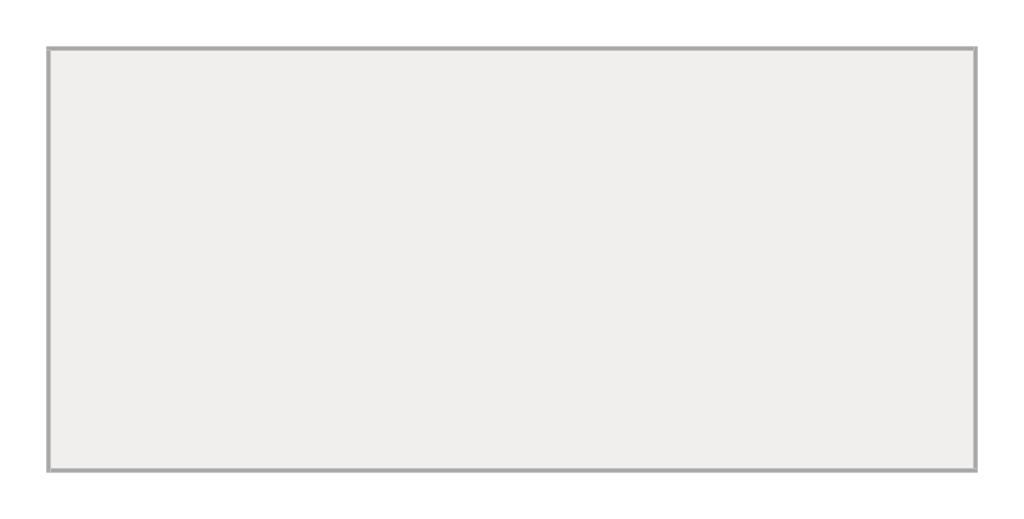
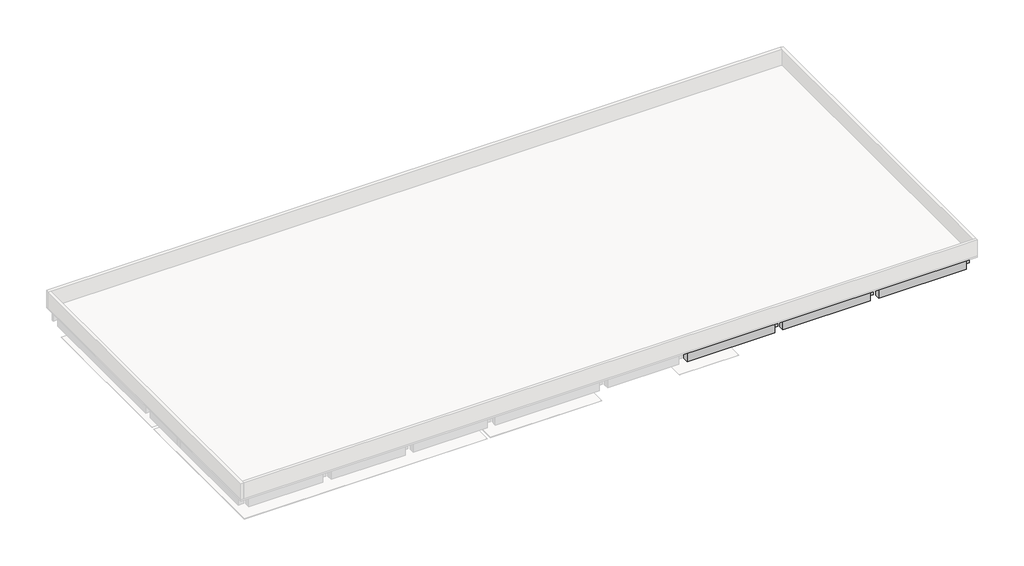
# One storey, part 2 of 2: 34 beams.
"""IFC4 building model written with IfcOpenShell, lengths in millimetres."""

from ifc_helpers import new_model, si_unit, frame, origin, place, context, project, spatial, polyline, outline, extrude, faceted_brep, element, save

model = new_model("IFC4")

# Units and contexts
model_context = context("Model", 3, world=origin())
ifc_project = project(units=[si_unit("LENGTHUNIT", "METRE", prefix="MILLI")], contexts=[model_context])

# Site, building, storey
site = spatial("IfcSite", under=ifc_project)
building = spatial("IfcBuilding", under=site)
storey = spatial("IfcBuildingStorey", under=building, Name="TOC", Elevation=7650.0)

# Beams
placement = place(None, origin())
element("IfcBeam", 1, ObjectType="RC Beam_Rectangular : H_SB_ACB_B400xH900", at=placement, inside=storey, context=model_context, shape_type="Brep", body=[
    faceted_brep([(32124.7, 12116.5208589, 6750.0), (32124.7, 12116.5208589, 7549.0), (31724.7, 12116.5208589, 7549.0), (26324.7, 12116.5208589, 7549.0), (26324.7, 12116.5208589, 6750.0), (31724.7, 12116.5208589, 6750.0), (32124.7, 12516.5208589, 6750.0), (26324.7, 12516.5208589, 6750.0), (31724.7, 12516.5208589, 6750.0), (32124.7, 12516.5208589, 7549.0), (26324.7, 12516.5208589, 7549.0), (31724.7, 12516.5208589, 7549.0)], [[[0, 1, 2, 3, 4, 5]], [[6, 0, 5, 4, 7, 8]], [[9, 6, 8, 7, 10, 11]], [[1, 9, 11, 10, 3, 2]], [[0, 6, 9, 1]], [[4, 3, 10, 7]]]),
])
element("IfcBeam", 2, ObjectType="RC Beam_Rectangular : H_SB_ACB_B400xH900", at=placement, inside=storey, context=model_context, shape_type="Brep", body=[
    faceted_brep([(39124.7, 12116.5208589, 6750.0), (39124.7, 12116.5208589, 7549.0), (38724.7, 12116.5208589, 7549.0), (32124.7, 12116.5208589, 7549.0), (32124.7, 12116.5208589, 6750.0), (38724.7, 12116.5208589, 6750.0), (39124.7, 12516.5208589, 6750.0), (32124.7, 12516.5208589, 6750.0), (38724.7, 12516.5208589, 6750.0), (39124.7, 12516.5208589, 7549.0), (32124.7, 12516.5208589, 7549.0), (38724.7, 12516.5208589, 7549.0)], [[[0, 1, 2, 3, 4, 5]], [[6, 0, 5, 4, 7, 8]], [[9, 6, 8, 7, 10, 11]], [[1, 9, 11, 10, 3, 2]], [[0, 6, 9, 1]], [[4, 3, 10, 7]]]),
])
element("IfcBeam", 3, ObjectType="RC Beam_Rectangular : H_SB_ACB_B400xH900", at=placement, inside=storey, context=model_context, shape_type="Brep", body=[
    faceted_brep([(46124.7, 12116.5208589, 6750.0), (46124.7, 12116.5208589, 7549.0), (45724.7, 12116.5208589, 7549.0), (39124.7, 12116.5208589, 7549.0), (39124.7, 12116.5208589, 6750.0), (45724.7, 12116.5208589, 6750.0), (46124.7, 12516.5208589, 6750.0), (39124.7, 12516.5208589, 6750.0), (45724.7, 12516.5208589, 6750.0), (46124.7, 12516.5208589, 7549.0), (39124.7, 12516.5208589, 7549.0), (45724.7, 12516.5208589, 7549.0)], [[[0, 1, 2, 3, 4, 5]], [[6, 0, 5, 4, 7, 8]], [[9, 6, 8, 7, 10, 11]], [[1, 9, 11, 10, 3, 2]], [[0, 6, 9, 1]], [[4, 3, 10, 7]]]),
])
element("IfcBeam", 4, ObjectType="RC Beam_Rectangular : H_SB_ACB_B400xH900", at=placement, inside=storey, context=model_context, shape_type="Brep", body=[
    faceted_brep([(53124.7, 12116.5208589, 6750.0), (53124.7, 12116.5208589, 7549.0), (52724.7, 12116.5208589, 7549.0), (46124.7, 12116.5208589, 7549.0), (46124.7, 12116.5208589, 6750.0), (52724.7, 12116.5208589, 6750.0), (53124.7, 12516.5208589, 6750.0), (46124.7, 12516.5208589, 6750.0), (52724.7, 12516.5208589, 6750.0), (53124.7, 12516.5208589, 7549.0), (46124.7, 12516.5208589, 7549.0), (52724.7, 12516.5208589, 7549.0)], [[[0, 1, 2, 3, 4, 5]], [[6, 0, 5, 4, 7, 8]], [[9, 6, 8, 7, 10, 11]], [[1, 9, 11, 10, 3, 2]], [[0, 6, 9, 1]], [[4, 3, 10, 7]]]),
])
element("IfcBeam", 5, ObjectType="RC Beam_Rectangular : H_SB_ACB_B400xH900", at=placement, inside=storey, context=model_context, shape_type="SweptSolid", body=[
    extrude(outline(polyline([(7500.0, 224.7), (6750.0, 224.7), (6750.0, 5624.7), (7500.0, 5624.7), (7500.0, 5724.7), (7549.0, 5724.7), (7549.0, 124.7), (7500.0, 124.7), (7500.0, 224.7)])), frame((0.0, 23816.5208589, 0.0), z_axis=(0.0, 1.0, 0.0), x_axis=(0.0, 0.0, 1.0)), (0.0, 0.0, 1.0), 400.0),
])
element("IfcBeam", 6, ObjectType="RC Beam_Rectangular : H_SB_ACB_B400xH900", at=placement, inside=storey, context=model_context, shape_type="SweptSolid", body=[
    extrude(outline(polyline([(7500.0, 6224.7), (6750.0, 6224.7), (6750.0, 11624.7), (7500.0, 11624.7), (7500.0, 11724.7), (7549.0, 11724.7), (7549.0, 6124.7), (7500.0, 6124.7), (7500.0, 6224.7)])), frame((0.0, 23816.5208589, 0.0), z_axis=(0.0, 1.0, 0.0), x_axis=(0.0, 0.0, 1.0)), (0.0, 0.0, 1.0), 400.0),
])
element("IfcBeam", 7, ObjectType="RC Beam_Rectangular : H_SB_ACB_B400xH900", at=placement, inside=storey, context=model_context, shape_type="SweptSolid", body=[
    extrude(outline(polyline([(7500.0, 12224.7), (6750.0, 12224.7), (6750.0, 17624.7), (7500.0, 17624.7), (7500.0, 17724.7), (7549.0, 17724.7), (7549.0, 12124.7), (7500.0, 12124.7), (7500.0, 12224.7)])), frame((0.0, 23816.5208589, 0.0), z_axis=(0.0, 1.0, 0.0), x_axis=(0.0, 0.0, 1.0)), (0.0, 0.0, 1.0), 400.0),
])
element("IfcBeam", 8, ObjectType="RC Beam_Rectangular : H_SB_ACB_B400xH900", at=placement, inside=storey, context=model_context, shape_type="SweptSolid", body=[
    extrude(outline(polyline([(7500.0, 18224.7), (6750.0, 18224.7), (6750.0, 25824.7), (7500.0, 25824.7), (7500.0, 25924.7), (7549.0, 25924.7), (7549.0, 18124.7), (7500.0, 18124.7), (7500.0, 18224.7)])), frame((0.0, 23816.5208589, 0.0), z_axis=(0.0, 1.0, 0.0), x_axis=(0.0, 0.0, 1.0)), (0.0, 0.0, 1.0), 400.0),
])
element("IfcBeam", 9, ObjectType="RC Beam_Rectangular : H_SB_ACB_B400xH900", at=placement, inside=storey, context=model_context, shape_type="SweptSolid", body=[
    extrude(outline(polyline([(7500.0, 26424.7), (6750.0, 26424.7), (6750.0, 31624.7), (7500.0, 31624.7), (7500.0, 31724.7), (7549.0, 31724.7), (7549.0, 26324.7), (7500.0, 26324.7), (7500.0, 26424.7)])), frame((0.0, 23816.5208589, 0.0), z_axis=(0.0, 1.0, 0.0), x_axis=(0.0, 0.0, 1.0)), (0.0, 0.0, 1.0), 400.0),
])
element("IfcBeam", 10, ObjectType="RC Beam_Rectangular : H_SB_ACB_B400xH900", at=placement, inside=storey, context=model_context, shape_type="SweptSolid", body=[
    extrude(outline(polyline([(7500.0, 32224.7), (6750.0, 32224.7), (6750.0, 38624.7), (7500.0, 38624.7), (7500.0, 38724.7), (7549.0, 38724.7), (7549.0, 32124.7), (7500.0, 32124.7), (7500.0, 32224.7)])), frame((0.0, 23816.5208589, 0.0), z_axis=(0.0, 1.0, 0.0), x_axis=(0.0, 0.0, 1.0)), (0.0, 0.0, 1.0), 400.0),
])
element("IfcBeam", 11, ObjectType="RC Beam_Rectangular : H_SB_ACB_B400xH900", at=placement, inside=storey, context=model_context, shape_type="SweptSolid", body=[
    extrude(outline(polyline([(7500.0, 39224.7), (6750.0, 39224.7), (6750.0, 45624.7), (7500.0, 45624.7), (7500.0, 45724.7), (7549.0, 45724.7), (7549.0, 39124.7), (7500.0, 39124.7), (7500.0, 39224.7)])), frame((0.0, 23816.5208589, 0.0), z_axis=(0.0, 1.0, 0.0), x_axis=(0.0, 0.0, 1.0)), (0.0, 0.0, 1.0), 400.0),
])
element("IfcBeam", 12, ObjectType="RC Beam_Rectangular : H_SB_ACB_B400xH900", at=placement, inside=storey, context=model_context, shape_type="SweptSolid", body=[
    extrude(outline(polyline([(7500.0, 46224.7), (6750.0, 46224.7), (6750.0, 52624.7), (7500.0, 52624.7), (7500.0, 52724.7), (7549.0, 52724.7), (7549.0, 46124.7), (7500.0, 46124.7), (7500.0, 46224.7)])), frame((0.0, 23816.5208589, 0.0), z_axis=(0.0, 1.0, 0.0), x_axis=(0.0, 0.0, 1.0)), (0.0, 0.0, 1.0), 400.0),
])
element("IfcBeam", 13, ObjectType="RC Beam_Rectangular : H_SB_ACB_B400xH900", at=placement, inside=storey, context=model_context, shape_type="Brep", body=[
    faceted_brep([(26424.7, 8216.5208589, 7500.0), (26424.7, 8216.5208589, 6750.0), (31624.7, 8216.5208589, 6750.0), (31624.7, 8216.5208589, 7500.0), (31724.7, 8216.5208589, 7500.0), (32124.7, 8216.5208589, 7500.0), (32124.7, 8216.5208589, 7549.0), (31724.7, 8216.5208589, 7549.0), (26324.7, 8216.5208589, 7549.0), (26324.7, 8216.5208589, 7500.0), (26424.7, 8616.5208589, 6750.0), (31624.7, 8616.5208589, 6750.0), (26424.7, 8616.5208589, 7500.0), (26324.7, 8616.5208589, 7500.0), (26324.7, 8616.5208589, 7549.0), (31724.7, 8616.5208589, 7549.0), (32124.7, 8616.5208589, 7549.0), (32124.7, 8616.5208589, 7500.0), (31724.7, 8616.5208589, 7500.0), (31624.7, 8616.5208589, 7500.0)], [[[0, 1, 2, 3, 4, 5, 6, 7, 8, 9]], [[1, 10, 11, 2]], [[10, 12, 13, 14, 15, 16, 17, 18, 19, 11]], [[1, 0, 12, 10]], [[0, 9, 13, 12]], [[19, 3, 2, 11]], [[3, 19, 18, 17, 5, 4]], [[8, 7, 6, 16, 15, 14]], [[16, 6, 5, 17]], [[8, 14, 13, 9]]]),
])
element("IfcBeam", 14, ObjectType="RC Beam_Rectangular : H_SB_ACB_B400xH900", at=placement, inside=storey, context=model_context, shape_type="Brep", body=[
    faceted_brep([(32224.7, 8216.5208589, 7500.0), (32224.7, 8216.5208589, 6750.0), (38624.7, 8216.5208589, 6750.0), (38624.7, 8216.5208589, 7500.0), (38724.7, 8216.5208589, 7500.0), (39124.7, 8216.5208589, 7500.0), (39124.7, 8216.5208589, 7549.0), (38724.7, 8216.5208589, 7549.0), (32124.7, 8216.5208589, 7549.0), (32124.7, 8216.5208589, 7500.0), (32224.7, 8616.5208589, 6750.0), (38624.7, 8616.5208589, 6750.0), (32224.7, 8616.5208589, 7500.0), (32124.7, 8616.5208589, 7500.0), (32124.7, 8616.5208589, 7549.0), (38724.7, 8616.5208589, 7549.0), (39124.7, 8616.5208589, 7549.0), (39124.7, 8616.5208589, 7500.0), (38724.7, 8616.5208589, 7500.0), (38624.7, 8616.5208589, 7500.0)], [[[0, 1, 2, 3, 4, 5, 6, 7, 8, 9]], [[1, 10, 11, 2]], [[10, 12, 13, 14, 15, 16, 17, 18, 19, 11]], [[1, 0, 12, 10]], [[0, 9, 13, 12]], [[19, 3, 2, 11]], [[3, 19, 18, 17, 5, 4]], [[8, 7, 6, 16, 15, 14]], [[16, 6, 5, 17]], [[8, 14, 13, 9]]]),
])
element("IfcBeam", 15, ObjectType="RC Beam_Rectangular : H_SB_ACB_B400xH900", at=placement, inside=storey, context=model_context, shape_type="Brep", body=[
    faceted_brep([(39224.7, 8216.5208589, 7500.0), (39224.7, 8216.5208589, 6750.0), (45624.7, 8216.5208589, 6750.0), (45624.7, 8216.5208589, 7500.0), (45724.7, 8216.5208589, 7500.0), (46124.7, 8216.5208589, 7500.0), (46124.7, 8216.5208589, 7549.0), (45724.7, 8216.5208589, 7549.0), (39124.7, 8216.5208589, 7549.0), (39124.7, 8216.5208589, 7500.0), (39224.7, 8616.5208589, 6750.0), (45624.7, 8616.5208589, 6750.0), (39224.7, 8616.5208589, 7500.0), (39124.7, 8616.5208589, 7500.0), (39124.7, 8616.5208589, 7549.0), (45724.7, 8616.5208589, 7549.0), (46124.7, 8616.5208589, 7549.0), (46124.7, 8616.5208589, 7500.0), (45724.7, 8616.5208589, 7500.0), (45624.7, 8616.5208589, 7500.0)], [[[0, 1, 2, 3, 4, 5, 6, 7, 8, 9]], [[1, 10, 11, 2]], [[10, 12, 13, 14, 15, 16, 17, 18, 19, 11]], [[1, 0, 12, 10]], [[0, 9, 13, 12]], [[19, 3, 2, 11]], [[3, 19, 18, 17, 5, 4]], [[8, 7, 6, 16, 15, 14]], [[16, 6, 5, 17]], [[8, 14, 13, 9]]]),
])
element("IfcBeam", 16, ObjectType="RC Beam_Rectangular : H_SB_ACB_B400xH900", at=placement, inside=storey, context=model_context, shape_type="Brep", body=[
    faceted_brep([(46224.7, 8216.5208589, 7500.0), (46224.7, 8216.5208589, 6750.0), (52624.7, 8216.5208589, 6750.0), (52624.7, 8216.5208589, 7500.0), (52724.7, 8216.5208589, 7500.0), (53124.7, 8216.5208589, 7500.0), (53124.7, 8216.5208589, 7549.0), (52724.7, 8216.5208589, 7549.0), (46124.7, 8216.5208589, 7549.0), (46124.7, 8216.5208589, 7500.0), (46224.7, 8616.5208589, 6750.0), (52624.7, 8616.5208589, 6750.0), (46224.7, 8616.5208589, 7500.0), (46124.7, 8616.5208589, 7500.0), (46124.7, 8616.5208589, 7549.0), (52724.7, 8616.5208589, 7549.0), (53124.7, 8616.5208589, 7549.0), (53124.7, 8616.5208589, 7500.0), (52724.7, 8616.5208589, 7500.0), (52624.7, 8616.5208589, 7500.0)], [[[0, 1, 2, 3, 4, 5, 6, 7, 8, 9]], [[1, 10, 11, 2]], [[10, 12, 13, 14, 15, 16, 17, 18, 19, 11]], [[1, 0, 12, 10]], [[0, 9, 13, 12]], [[19, 3, 2, 11]], [[3, 19, 18, 17, 5, 4]], [[8, 7, 6, 16, 15, 14]], [[16, 6, 5, 17]], [[8, 14, 13, 9]]]),
])
element("IfcBeam", 17, ObjectType="RC Beam_Rectangular : H_SB_ACB_B400xH900", at=placement, inside=storey, context=model_context, shape_type="Brep", body=[
    faceted_brep([(32224.7, 416.5208589, 7500.0), (32224.7, 416.5208589, 6750.0), (38624.7, 416.5208589, 6750.0), (38624.7, 416.5208589, 7500.0), (39124.7, 416.5208589, 7500.0), (39124.7, 416.5208589, 7549.0), (32124.7, 416.5208589, 7549.0), (32124.7, 416.5208589, 7500.0), (32224.7, 816.5208589, 6750.0), (38624.7, 816.5208589, 6750.0), (32224.7, 816.5208589, 7500.0), (32124.7, 816.5208589, 7500.0), (32124.7, 816.5208589, 7549.0), (38724.7, 816.5208589, 7549.0), (39124.7, 816.5208589, 7549.0), (39124.7, 816.5208589, 7500.0), (38724.7, 816.5208589, 7500.0), (38624.7, 816.5208589, 7500.0)], [[[0, 1, 2, 3, 4, 5, 6, 7]], [[1, 8, 9, 2]], [[8, 10, 11, 12, 13, 14, 15, 16, 17, 9]], [[8, 1, 0, 10]], [[11, 10, 0, 7]], [[17, 3, 2, 9]], [[3, 17, 16, 15, 4]], [[6, 5, 14, 13, 12]], [[14, 5, 4, 15]], [[6, 12, 11, 7]]]),
])
element("IfcBeam", 18, ObjectType="RC Beam_Rectangular : H_SB_ACB_B400xH900", at=placement, inside=storey, context=model_context, shape_type="Brep", body=[
    faceted_brep([(39224.7, 416.5208589, 7500.0), (39224.7, 416.5208589, 6750.0), (45624.7, 416.5208589, 6750.0), (45624.7, 416.5208589, 7500.0), (46124.7, 416.5208589, 7500.0), (46124.7, 416.5208589, 7549.0), (39124.7, 416.5208589, 7549.0), (39124.7, 416.5208589, 7500.0), (39224.7, 816.5208589, 6750.0), (45624.7, 816.5208589, 6750.0), (39224.7, 816.5208589, 7500.0), (39124.7, 816.5208589, 7500.0), (39124.7, 816.5208589, 7549.0), (45724.7, 816.5208589, 7549.0), (46124.7, 816.5208589, 7549.0), (46124.7, 816.5208589, 7500.0), (45724.7, 816.5208589, 7500.0), (45624.7, 816.5208589, 7500.0)], [[[0, 1, 2, 3, 4, 5, 6, 7]], [[1, 8, 9, 2]], [[8, 10, 11, 12, 13, 14, 15, 16, 17, 9]], [[8, 1, 0, 10]], [[11, 10, 0, 7]], [[17, 3, 2, 9]], [[3, 17, 16, 15, 4]], [[6, 5, 14, 13, 12]], [[14, 5, 4, 15]], [[6, 12, 11, 7]]]),
])
element("IfcBeam", 19, ObjectType="RC Beam_Rectangular : H_SB_ACB_B400xH900", at=placement, inside=storey, context=model_context, shape_type="Brep", body=[
    faceted_brep([(46224.7, 416.5208589, 7500.0), (46224.7, 416.5208589, 6750.0), (52624.7, 416.5208589, 6750.0), (52624.7, 416.5208589, 7500.0), (53124.7, 416.5208589, 7500.0), (53124.7, 416.5208589, 7549.0), (46124.7, 416.5208589, 7549.0), (46124.7, 416.5208589, 7500.0), (46224.7, 816.5208589, 6750.0), (52624.7, 816.5208589, 6750.0), (46224.7, 816.5208589, 7500.0), (46124.7, 816.5208589, 7500.0), (46124.7, 816.5208589, 7549.0), (52724.7, 816.5208589, 7549.0), (53124.7, 816.5208589, 7549.0), (53124.7, 816.5208589, 7500.0), (52724.7, 816.5208589, 7500.0), (52624.7, 816.5208589, 7500.0)], [[[0, 1, 2, 3, 4, 5, 6, 7]], [[1, 8, 9, 2]], [[8, 10, 11, 12, 13, 14, 15, 16, 17, 9]], [[8, 1, 0, 10]], [[11, 10, 0, 7]], [[17, 3, 2, 9]], [[3, 17, 16, 15, 4]], [[6, 5, 14, 13, 12]], [[14, 5, 4, 15]], [[6, 12, 11, 7]]]),
])
element("IfcBeam", 20, ObjectType="RC Beam_Rectangular : H_SB_ACB_B400xH900", at=placement, inside=storey, context=model_context, shape_type="Brep", body=[
    faceted_brep([(6124.7, 24429.2208589, 6750.0), (5724.7, 24429.2208589, 6750.0), (5724.7, 24429.2208589, 7549.0), (6124.7, 24429.2208589, 7549.0), (6124.7, 12616.5208589, 7500.0), (6124.7, 12616.5208589, 6750.0), (6124.7, 23716.5208589, 6750.0), (6124.7, 23716.5208589, 7500.0), (6124.7, 23816.5208589, 7500.0), (6124.7, 24216.5208589, 7500.0), (6124.7, 24316.5208589, 7500.0), (6124.7, 24316.5208589, 6750.0), (6124.7, 24216.5208589, 7549.0), (6124.7, 23816.5208589, 7549.0), (6124.7, 12516.5208589, 7549.0), (6124.7, 12516.5208589, 7500.0), (5724.7, 24316.5208589, 6750.0), (5724.7, 24316.5208589, 7500.0), (5724.7, 24216.5208589, 7500.0), (5724.7, 23816.5208589, 7500.0), (5724.7, 23716.5208589, 7500.0), (5724.7, 23716.5208589, 6750.0), (5724.7, 12616.5208589, 6750.0), (5724.7, 12616.5208589, 7500.0), (5724.7, 12516.5208589, 7500.0), (5724.7, 12516.5208589, 7549.0), (5724.7, 23816.5208589, 7549.0), (5724.7, 24216.5208589, 7549.0)], [[[0, 1, 2, 3]], [[4, 5, 6, 7, 8, 9, 10, 11, 0, 3, 12, 13, 14, 15]], [[1, 0, 11, 16]], [[2, 1, 16, 17, 18, 19, 20, 21, 22, 23, 24, 25, 26, 27]], [[24, 15, 14, 25]], [[5, 4, 23, 22]], [[4, 15, 24, 23]], [[20, 7, 6, 21]], [[7, 20, 19, 18, 17, 10, 9, 8]], [[3, 2, 27, 26, 25, 14, 13, 12]], [[10, 17, 16, 11]], [[5, 22, 21, 6]]]),
])
element("IfcBeam", 21, ObjectType="RC Beam_Rectangular : H_SB_ACB_B400xH900", at=placement, inside=storey, context=model_context, shape_type="Brep", body=[
    faceted_brep([(12124.7, 24429.2208589, 6750.0), (11724.7, 24429.2208589, 6750.0), (11724.7, 24429.2208589, 7549.0), (12124.7, 24429.2208589, 7549.0), (12124.7, 12616.5208589, 7500.0), (12124.7, 12616.5208589, 6750.0), (12124.7, 23716.5208589, 6750.0), (12124.7, 23716.5208589, 7500.0), (12124.7, 23816.5208589, 7500.0), (12124.7, 24216.5208589, 7500.0), (12124.7, 24316.5208589, 7500.0), (12124.7, 24316.5208589, 6750.0), (12124.7, 24216.5208589, 7549.0), (12124.7, 23816.5208589, 7549.0), (12124.7, 12516.5208589, 7549.0), (12124.7, 12516.5208589, 7500.0), (11724.7, 24316.5208589, 6750.0), (11724.7, 24316.5208589, 7500.0), (11724.7, 24216.5208589, 7500.0), (11724.7, 23816.5208589, 7500.0), (11724.7, 23716.5208589, 7500.0), (11724.7, 23716.5208589, 6750.0), (11724.7, 12616.5208589, 6750.0), (11724.7, 12616.5208589, 7500.0), (11724.7, 12516.5208589, 7500.0), (11724.7, 12516.5208589, 7549.0), (11724.7, 23816.5208589, 7549.0), (11724.7, 24216.5208589, 7549.0)], [[[0, 1, 2, 3]], [[4, 5, 6, 7, 8, 9, 10, 11, 0, 3, 12, 13, 14, 15]], [[1, 0, 11, 16]], [[2, 1, 16, 17, 18, 19, 20, 21, 22, 23, 24, 25, 26, 27]], [[24, 15, 14, 25]], [[5, 4, 23, 22]], [[4, 15, 24, 23]], [[20, 7, 6, 21]], [[7, 20, 19, 18, 17, 10, 9, 8]], [[3, 2, 27, 26, 25, 14, 13, 12]], [[10, 17, 16, 11]], [[5, 22, 21, 6]]]),
])
element("IfcBeam", 22, ObjectType="RC Beam_Rectangular : H_SB_ACB_B400xH900", at=placement, inside=storey, context=model_context, shape_type="Brep", body=[
    faceted_brep([(18124.7, 24429.2208589, 6750.0), (17724.7, 24429.2208589, 6750.0), (17724.7, 24429.2208589, 7549.0), (18124.7, 24429.2208589, 7549.0), (18124.7, 12616.5208589, 7500.0), (18124.7, 12616.5208589, 6750.0), (18124.7, 23716.5208589, 6750.0), (18124.7, 23716.5208589, 7500.0), (18124.7, 23816.5208589, 7500.0), (18124.7, 24216.5208589, 7500.0), (18124.7, 24316.5208589, 7500.0), (18124.7, 24316.5208589, 6750.0), (18124.7, 24216.5208589, 7549.0), (18124.7, 23816.5208589, 7549.0), (18124.7, 12516.5208589, 7549.0), (18124.7, 12516.5208589, 7500.0), (17724.7, 24316.5208589, 6750.0), (17724.7, 24316.5208589, 7500.0), (17724.7, 24216.5208589, 7500.0), (17724.7, 23816.5208589, 7500.0), (17724.7, 23716.5208589, 7500.0), (17724.7, 23716.5208589, 6750.0), (17724.7, 12616.5208589, 6750.0), (17724.7, 12616.5208589, 7500.0), (17724.7, 12516.5208589, 7500.0), (17724.7, 12516.5208589, 7549.0), (17724.7, 23816.5208589, 7549.0), (17724.7, 24216.5208589, 7549.0)], [[[0, 1, 2, 3]], [[4, 5, 6, 7, 8, 9, 10, 11, 0, 3, 12, 13, 14, 15]], [[1, 0, 11, 16]], [[2, 1, 16, 17, 18, 19, 20, 21, 22, 23, 24, 25, 26, 27]], [[24, 15, 14, 25]], [[5, 4, 23, 22]], [[4, 15, 24, 23]], [[20, 7, 6, 21]], [[7, 20, 19, 18, 17, 10, 9, 8]], [[3, 2, 27, 26, 25, 14, 13, 12]], [[10, 17, 16, 11]], [[5, 22, 21, 6]]]),
])
element("IfcBeam", 23, ObjectType="RC Beam_Rectangular : H_SB_ACB_B400xH900", at=placement, inside=storey, context=model_context, shape_type="Brep", body=[
    faceted_brep([(26324.7, 24429.2208589, 6750.0), (25924.7, 24429.2208589, 6750.0), (25924.7, 24429.2208589, 7549.0), (26324.7, 24429.2208589, 7549.0), (26324.7, 24216.5208589, 7549.0), (26324.7, 23816.5208589, 7549.0), (26324.7, 12516.5208589, 7549.0), (26324.7, 12516.5208589, 6750.0), (26324.7, 23716.5208589, 6750.0), (26324.7, 23716.5208589, 7500.0), (26324.7, 23816.5208589, 7500.0), (26324.7, 24216.5208589, 7500.0), (26324.7, 24316.5208589, 7500.0), (26324.7, 24316.5208589, 6750.0), (25924.7, 24316.5208589, 6750.0), (25924.7, 12516.5208589, 6750.0), (25924.7, 12516.5208589, 7549.0), (25924.7, 23816.5208589, 7549.0), (25924.7, 24216.5208589, 7549.0), (25924.7, 24316.5208589, 7500.0), (25924.7, 24216.5208589, 7500.0), (25924.7, 23816.5208589, 7500.0), (25924.7, 23716.5208589, 7500.0), (25924.7, 23716.5208589, 6750.0)], [[[0, 1, 2, 3]], [[0, 3, 4, 5, 6, 7, 8, 9, 10, 11, 12, 13]], [[1, 0, 13, 14]], [[15, 16, 17, 18, 2, 1, 14, 19, 20, 21, 22, 23]], [[15, 7, 6, 16]], [[22, 9, 8, 23]], [[9, 22, 21, 20, 19, 12, 11, 10]], [[3, 2, 18, 17, 16, 6, 5, 4]], [[12, 19, 14, 13]], [[7, 15, 23, 8]]]),
])
element("IfcBeam", 24, ObjectType="RC Beam_Rectangular : H_SB_ACB_B400xH900", at=placement, inside=storey, context=model_context, shape_type="SweptSolid", body=[
    extrude(outline(polyline([(12116.5208589, 7549.0), (12116.5208589, 6750.0), (8716.5208589, 6750.0), (8716.5208589, 7500.0), (8616.5208589, 7500.0), (8616.5208589, 7549.0), (12116.5208589, 7549.0)])), frame((31724.7, 0.0, 0.0), z_axis=(1.0, 0.0, 0.0), x_axis=(0.0, 1.0, 0.0)), (0.0, 0.0, 1.0), 400.0),
])
element("IfcBeam", 25, ObjectType="RC Beam_Rectangular : H_SB_ACB_B400xH900", at=placement, inside=storey, context=model_context, shape_type="Brep", body=[
    faceted_brep([(32124.7, 24429.2208589, 6750.0), (31724.7, 24429.2208589, 6750.0), (31724.7, 24429.2208589, 7549.0), (32124.7, 24429.2208589, 7549.0), (32124.7, 24216.5208589, 7549.0), (32124.7, 23816.5208589, 7549.0), (32124.7, 12516.5208589, 7549.0), (32124.7, 12516.5208589, 6750.0), (32124.7, 23716.5208589, 6750.0), (32124.7, 23716.5208589, 7500.0), (32124.7, 23816.5208589, 7500.0), (32124.7, 24216.5208589, 7500.0), (32124.7, 24316.5208589, 7500.0), (32124.7, 24316.5208589, 6750.0), (31724.7, 24316.5208589, 6750.0), (31724.7, 12516.5208589, 6750.0), (31724.7, 12516.5208589, 7549.0), (31724.7, 23816.5208589, 7549.0), (31724.7, 24216.5208589, 7549.0), (31724.7, 24316.5208589, 7500.0), (31724.7, 24216.5208589, 7500.0), (31724.7, 23816.5208589, 7500.0), (31724.7, 23716.5208589, 7500.0), (31724.7, 23716.5208589, 6750.0)], [[[0, 1, 2, 3]], [[0, 3, 4, 5, 6, 7, 8, 9, 10, 11, 12, 13]], [[1, 0, 13, 14]], [[15, 16, 17, 18, 2, 1, 14, 19, 20, 21, 22, 23]], [[15, 7, 6, 16]], [[22, 9, 8, 23]], [[9, 22, 21, 20, 19, 12, 11, 10]], [[3, 2, 18, 17, 16, 6, 5, 4]], [[12, 19, 14, 13]], [[7, 15, 23, 8]]]),
])
element("IfcBeam", 26, ObjectType="RC Beam_Rectangular : H_SB_ACB_B400xH900", at=placement, inside=storey, context=model_context, shape_type="SweptSolid", body=[
    extrude(outline(polyline([(8116.5208589, 7500.0), (8116.5208589, 6750.0), (916.5208589, 6750.0), (916.5208589, 7500.0), (816.5208589, 7500.0), (816.5208589, 7549.0), (8216.5208589, 7549.0), (8216.5208589, 7500.0), (8116.5208589, 7500.0)])), frame((38724.7, 0.0, 0.0), z_axis=(1.0, 0.0, 0.0), x_axis=(0.0, 1.0, 0.0)), (0.0, 0.0, 1.0), 400.0),
])
element("IfcBeam", 27, ObjectType="RC Beam_Rectangular : H_SB_ACB_B400xH900", at=placement, inside=storey, context=model_context, shape_type="SweptSolid", body=[
    extrude(outline(polyline([(12116.5208589, 7549.0), (12116.5208589, 6750.0), (8716.5208589, 6750.0), (8716.5208589, 7500.0), (8616.5208589, 7500.0), (8616.5208589, 7549.0), (12116.5208589, 7549.0)])), frame((38724.7, 0.0, 0.0), z_axis=(1.0, 0.0, 0.0), x_axis=(0.0, 1.0, 0.0)), (0.0, 0.0, 1.0), 400.0),
])
element("IfcBeam", 28, ObjectType="RC Beam_Rectangular : H_SB_ACB_B400xH900", at=placement, inside=storey, context=model_context, shape_type="Brep", body=[
    faceted_brep([(39124.7, 24429.2208589, 6750.0), (38724.7, 24429.2208589, 6750.0), (38724.7, 24429.2208589, 7549.0), (39124.7, 24429.2208589, 7549.0), (39124.7, 24216.5208589, 7549.0), (39124.7, 23816.5208589, 7549.0), (39124.7, 12516.5208589, 7549.0), (39124.7, 12516.5208589, 6750.0), (39124.7, 23716.5208589, 6750.0), (39124.7, 23716.5208589, 7500.0), (39124.7, 23816.5208589, 7500.0), (39124.7, 24216.5208589, 7500.0), (39124.7, 24316.5208589, 7500.0), (39124.7, 24316.5208589, 6750.0), (38724.7, 24316.5208589, 6750.0), (38724.7, 12516.5208589, 6750.0), (38724.7, 12516.5208589, 7549.0), (38724.7, 23816.5208589, 7549.0), (38724.7, 24216.5208589, 7549.0), (38724.7, 24316.5208589, 7500.0), (38724.7, 24216.5208589, 7500.0), (38724.7, 23816.5208589, 7500.0), (38724.7, 23716.5208589, 7500.0), (38724.7, 23716.5208589, 6750.0)], [[[0, 1, 2, 3]], [[0, 3, 4, 5, 6, 7, 8, 9, 10, 11, 12, 13]], [[1, 0, 13, 14]], [[15, 16, 17, 18, 2, 1, 14, 19, 20, 21, 22, 23]], [[15, 7, 6, 16]], [[22, 9, 8, 23]], [[9, 22, 21, 20, 19, 12, 11, 10]], [[3, 2, 18, 17, 16, 6, 5, 4]], [[12, 19, 14, 13]], [[7, 15, 23, 8]]]),
])
element("IfcBeam", 29, ObjectType="RC Beam_Rectangular : H_SB_ACB_B400xH900", at=placement, inside=storey, context=model_context, shape_type="SweptSolid", body=[
    extrude(outline(polyline([(8116.5208589, 7500.0), (8116.5208589, 6750.0), (916.5208589, 6750.0), (916.5208589, 7500.0), (816.5208589, 7500.0), (816.5208589, 7549.0), (8216.5208589, 7549.0), (8216.5208589, 7500.0), (8116.5208589, 7500.0)])), frame((45724.7, 0.0, 0.0), z_axis=(1.0, 0.0, 0.0), x_axis=(0.0, 1.0, 0.0)), (0.0, 0.0, 1.0), 400.0),
])
element("IfcBeam", 30, ObjectType="RC Beam_Rectangular : H_SB_ACB_B400xH900", at=placement, inside=storey, context=model_context, shape_type="SweptSolid", body=[
    extrude(outline(polyline([(12116.5208589, 7549.0), (12116.5208589, 6750.0), (8716.5208589, 6750.0), (8716.5208589, 7500.0), (8616.5208589, 7500.0), (8616.5208589, 7549.0), (12116.5208589, 7549.0)])), frame((45724.7, 0.0, 0.0), z_axis=(1.0, 0.0, 0.0), x_axis=(0.0, 1.0, 0.0)), (0.0, 0.0, 1.0), 400.0),
])
element("IfcBeam", 31, ObjectType="RC Beam_Rectangular : H_SB_ACB_B400xH900", at=placement, inside=storey, context=model_context, shape_type="Brep", body=[
    faceted_brep([(46124.7, 24429.2208589, 6750.0), (45724.7, 24429.2208589, 6750.0), (45724.7, 24429.2208589, 7549.0), (46124.7, 24429.2208589, 7549.0), (46124.7, 24216.5208589, 7549.0), (46124.7, 23816.5208589, 7549.0), (46124.7, 12516.5208589, 7549.0), (46124.7, 12516.5208589, 6750.0), (46124.7, 23716.5208589, 6750.0), (46124.7, 23716.5208589, 7500.0), (46124.7, 23816.5208589, 7500.0), (46124.7, 24216.5208589, 7500.0), (46124.7, 24316.5208589, 7500.0), (46124.7, 24316.5208589, 6750.0), (45724.7, 24316.5208589, 6750.0), (45724.7, 12516.5208589, 6750.0), (45724.7, 12516.5208589, 7549.0), (45724.7, 23816.5208589, 7549.0), (45724.7, 24216.5208589, 7549.0), (45724.7, 24316.5208589, 7500.0), (45724.7, 24216.5208589, 7500.0), (45724.7, 23816.5208589, 7500.0), (45724.7, 23716.5208589, 7500.0), (45724.7, 23716.5208589, 6750.0)], [[[0, 1, 2, 3]], [[0, 3, 4, 5, 6, 7, 8, 9, 10, 11, 12, 13]], [[1, 0, 13, 14]], [[15, 16, 17, 18, 2, 1, 14, 19, 20, 21, 22, 23]], [[15, 7, 6, 16]], [[22, 9, 8, 23]], [[9, 22, 21, 20, 19, 12, 11, 10]], [[3, 2, 18, 17, 16, 6, 5, 4]], [[12, 19, 14, 13]], [[7, 15, 23, 8]]]),
])
element("IfcBeam", 32, ObjectType="RC Beam_Rectangular : H_SB_ACB_B400xH900", at=placement, inside=storey, context=model_context, shape_type="SweptSolid", body=[
    extrude(outline(polyline([(8116.5208589, 7500.0), (8116.5208589, 6750.0), (916.5208589, 6750.0), (916.5208589, 7500.0), (816.5208589, 7500.0), (816.5208589, 7549.0), (8216.5208589, 7549.0), (8216.5208589, 7500.0), (8116.5208589, 7500.0)])), frame((52724.7, 0.0, 0.0), z_axis=(1.0, 0.0, 0.0), x_axis=(0.0, 1.0, 0.0)), (0.0, 0.0, 1.0), 400.0),
])
element("IfcBeam", 33, ObjectType="RC Beam_Rectangular : H_SB_ACB_B400xH900", at=placement, inside=storey, context=model_context, shape_type="SweptSolid", body=[
    extrude(outline(polyline([(12116.5208589, 7549.0), (12116.5208589, 6750.0), (8716.5208589, 6750.0), (8716.5208589, 7500.0), (8616.5208589, 7500.0), (8616.5208589, 7549.0), (12116.5208589, 7549.0)])), frame((52724.7, 0.0, 0.0), z_axis=(1.0, 0.0, 0.0), x_axis=(0.0, 1.0, 0.0)), (0.0, 0.0, 1.0), 400.0),
])
element("IfcBeam", 34, ObjectType="RC Beam_Rectangular : H_SB_ACB_B400xH900", at=placement, inside=storey, context=model_context, shape_type="Brep", body=[
    faceted_brep([(53124.7, 24429.2208589, 6750.0), (52724.7, 24429.2208589, 6750.0), (52724.7, 24429.2208589, 7549.0), (53124.7, 24429.2208589, 7549.0), (53124.7, 23716.5208589, 6750.0), (53124.7, 23716.5208589, 7500.0), (53124.7, 24316.5208589, 7500.0), (53124.7, 24316.5208589, 6750.0), (53124.7, 12516.5208589, 7549.0), (53124.7, 12516.5208589, 6750.0), (52724.7, 24316.5208589, 6750.0), (52724.7, 24316.5208589, 7500.0), (52724.7, 24216.5208589, 7500.0), (52724.7, 23816.5208589, 7500.0), (52724.7, 23716.5208589, 7500.0), (52724.7, 23716.5208589, 6750.0), (52724.7, 12516.5208589, 6750.0), (52724.7, 12516.5208589, 7549.0), (52724.7, 23816.5208589, 7549.0), (52724.7, 24216.5208589, 7549.0)], [[[0, 1, 2, 3]], [[4, 5, 6, 7, 0, 3, 8, 9]], [[1, 0, 7, 10]], [[11, 12, 13, 14, 15, 16, 17, 18, 19, 2, 1, 10]], [[4, 15, 14, 5]], [[14, 13, 12, 11, 6, 5]], [[9, 8, 17, 16]], [[3, 2, 19, 18, 17, 8]], [[6, 11, 10, 7]], [[15, 4, 9, 16]]]),
])

save(model, "model.ifc")

# Revit data of these elements
# Type "RC Beam_Rectangular : H_SB_ACB_B400xH900"
#   중앙부 하부근 = ""
#   중앙부 상부근 = ""
#   중앙부 보조근 = ""
#   중앙부 늑근 = ""
#   외단부 하부근 = ""
#   외단부 상부근 = ""
#   외단부 보조근 = ""
#   외단부 늑근 = ""
#   부호 = "TG3"
#   내단부 하부근 = ""
#   내단부 상부근 = ""
#   내단부 보조근 = ""
#   내단부 늑근 = ""
#   ALL 하부근 = "3-D20"
#   ALL 상부근 = "3-D20"
#   ALL 보조근 = ""
#   ALL 늑근 = "2-D10 @120"
#   Width = 400.000 mm
#   Height = 900.000 mm
#   Length [instance default] = 1524.000 mm
#   b = 400.000 mm
#   h = 900.000 mm
#   hec_material3 [instance default] = none
#   hec_material2 [instance default] = none
#   hec_material1 [instance default] = none
#   Structural Material [instance default] = none
#   Assembly Code = ""
# Elements 1, 2, 3, 4, 5, 6, 7, 8, 9, 10, 11, 12, 13, 14, 15, 16, 17, 18, 19, 20, 21, 22, 23, 24, 25, 26, 27, 28, 29, 30, 31, 32, 33, 34 (IfcBeam, "RC Beam_Rectangular : H_SB_ACB_B400xH900")
#   hec_material3 = none
#   hec_material2 = none
#   hec_material1 = none
#   Structural Material = none
#   Phase Created = New Construction
